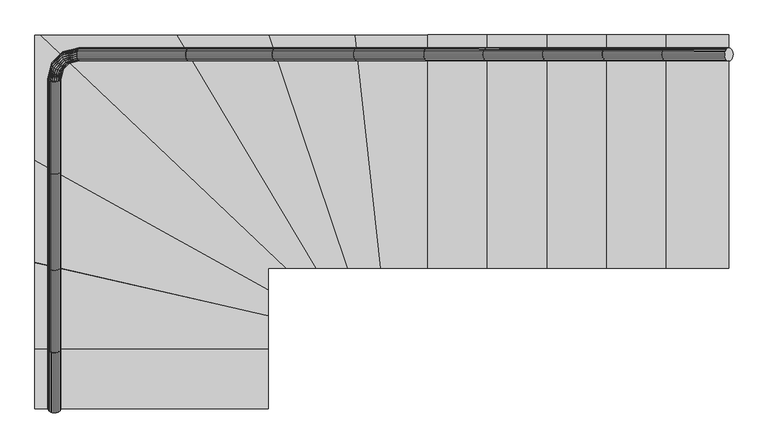
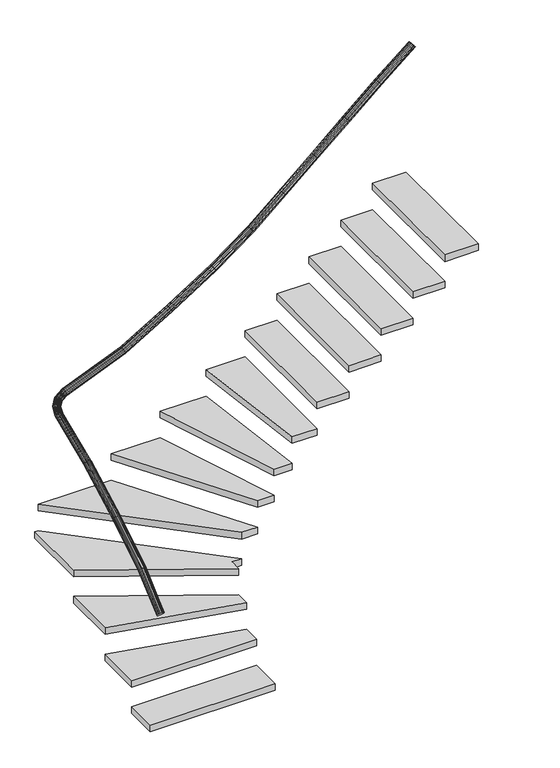
"""IFC4 building model written with IfcOpenShell, lengths in millimetres: stair geometry, 0_3d."""

from ifc_helpers import new_model, si_unit, frame, origin, origin_with_axes, place, context, project, spatial, polyline, outline, extrude, faceted_brep, source, transform, mapped, element, save


def stair_5eab08e0(model_context):
    return source(origin(), model_context, "Body", "SolidModel", [
        faceted_brep([(1247.9277886, 1358.1947934, 2262.9627611), (1243.4067036, 1356.9712063, 2269.5592366), (1238.8856187, 1358.1947934, 2276.1557121), (1234.8070891, 1361.7457815, 2282.1064787), (1231.5703496, 1367.276575, 2286.8290337), (1229.492235, 1374.2457815, 2289.8611007), (1228.7761655, 1381.9712063, 2290.9058798), (1229.492235, 1389.6966312, 2289.8611007), (1231.5703496, 1396.6658376, 2286.8290337), (1234.8070891, 1402.1966312, 2282.1064787), (1238.8856187, 1405.7476192, 2276.1557121), (1243.4067036, 1406.9712063, 2269.5592366), (1247.9277886, 1405.7476192, 2262.9627611), (1252.0063182, 1402.1966312, 2257.0119945), (1255.2430577, 1396.6658376, 2252.2894395), (1257.3211723, 1389.6966312, 2249.2573725), (1258.0372418, 1381.9712063, 2248.2125934), (1257.3211723, 1374.2457815, 2249.2573725), (1255.2430577, 1367.276575, 2252.2894395), (1252.0063182, 1361.7457815, 2257.0119945), (1509.5997401, 1358.1947934, 2475.8009775), (1514.6018366, 1356.9712063, 2469.5592366), (1519.6039331, 1358.1947934, 2463.3174957), (1524.1163895, 1361.7457815, 2457.6867399), (1527.6974952, 1367.276575, 2453.2181468), (1529.9967066, 1374.2457815, 2450.3491334), (1530.7889608, 1381.9712063, 2449.3605388), (1529.9967066, 1389.6966312, 2450.3491334), (1527.6974952, 1396.6658376, 2453.2181468), (1524.1163895, 1402.1966312, 2457.6867399), (1519.6039331, 1405.7476192, 2463.3174957), (1514.6018366, 1406.9712063, 2469.5592366), (1509.5997401, 1405.7476192, 2475.8009775), (1505.0872837, 1402.1966312, 2481.4317333), (1501.506178, 1396.6658376, 2485.9003264), (1499.2069666, 1389.6966312, 2488.7693398), (1498.4147124, 1381.9712063, 2489.7579344), (1499.2069666, 1374.2457815, 2488.7693398), (1501.506178, 1367.276575, 2485.9003264), (1505.0872837, 1361.7457815, 2481.4317333)], [[[0, 1, 2, 3, 4, 5, 6, 7, 8, 9, 10, 11, 12, 13, 14, 15, 16, 17, 18, 19]], [[20, 21, 22, 23, 24, 25, 26, 27, 28, 29, 30, 31, 32, 33, 34, 35, 36, 37, 38, 39]], [[2, 1, 21, 20]], [[3, 2, 20, 39]], [[4, 3, 39, 38]], [[5, 4, 38, 37]], [[6, 5, 37, 36]], [[7, 6, 36, 35]], [[8, 7, 35, 34]], [[9, 8, 34, 33]], [[10, 9, 33, 32]], [[11, 10, 32, 31]], [[12, 11, 31, 30]], [[13, 12, 30, 29]], [[14, 13, 29, 28]], [[15, 14, 28, 27]], [[16, 15, 27, 26]], [[17, 16, 26, 25]], [[18, 17, 25, 24]], [[19, 18, 24, 23]], [[0, 19, 23, 22]], [[1, 0, 22, 21]]]),
        extrude(outline(polyline([(1514.6018366, 1456.9712063), (1744.6018366, 1456.9712063), (1744.6018366, 556.9712063), (1514.6018366, 556.9712063), (1514.6018366, 1456.9712063)])), frame((0.0, 0.0, 1600.0), z_axis=(0.0, 0.0, 1.0), x_axis=(1.0, 0.0, 0.0)), (0.0, 0.0, 1.0), 50.0),
        extrude(outline(polyline([(0.0, 246.9712063), (0.0, 579.9383967), (900.0, 374.004016), (900.0, 246.9712063), (0.0, 246.9712063)])), frame((0.0, 0.0, 200.0), z_axis=(0.0, 0.0, 1.0), x_axis=(1.0, 0.0, 0.0)), (0.0, 0.0, 1.0), 50.0),
        extrude(outline(polyline([(2434.6018366, 1456.9712063), (2675.6316793, 1456.9712063), (2675.6316793, 556.9712063), (2434.6018366, 556.9712063), (2434.6018366, 1456.9712063)])), frame((0.0, 0.0, 2400.0), z_axis=(0.0, 0.0, 1.0), x_axis=(1.0, 0.0, 0.0)), (0.0, 0.0, 1.0), 50.0),
        extrude(outline(polyline([(548.3198618, 1456.9712063), (903.6283904, 1456.9712063), (1205.5752828, 556.9712063), (1084.8542159, 556.9712063), (548.3198618, 1456.9712063)])), frame((0.0, 0.0, 1000.0), z_axis=(0.0, 0.0, 1.0), x_axis=(1.0, 0.0, 0.0)), (0.0, 0.0, 1.0), 50.0),
        extrude(outline(polyline([(2204.6018366, 1456.9712063), (2434.6018366, 1456.9712063), (2434.6018366, 556.9712063), (2204.6018366, 556.9712063), (2204.6018366, 1456.9712063)])), frame((0.0, 0.0, 2200.0), z_axis=(0.0, 0.0, 1.0), x_axis=(1.0, 0.0, 0.0)), (0.0, 0.0, 1.0), 50.0),
        extrude(outline(polyline([(903.6283904, 1456.9712063), (1235.167677, 1456.9712063), (1334.0359962, 556.9712063), (1205.5752828, 556.9712063), (903.6283904, 1456.9712063)])), frame((0.0, 0.0, 1200.0), z_axis=(0.0, 0.0, 1.0), x_axis=(1.0, 0.0, 0.0)), (0.0, 0.0, 1.0), 50.0),
        faceted_brep([(98.7764129, 935.1107738, 1462.3430272), (100.0, 931.6520604, 1469.5592366), (98.7764129, 928.193347, 1476.775446), (95.2254249, 925.0731965, 1483.2852826), (89.6946313, 922.5970311, 1488.4515182), (82.7254249, 921.0072351, 1491.7684456), (75.0, 920.4594287, 1492.9113809), (67.2745751, 921.0072351, 1491.7684456), (60.3053687, 922.5970311, 1488.4515182), (54.7745751, 925.0731965, 1483.2852826), (51.2235871, 928.193347, 1476.775446), (50.0, 931.6520604, 1469.5592366), (51.2235871, 935.1107738, 1462.3430272), (54.7745751, 938.2309242, 1455.8331906), (60.3053687, 940.7070896, 1450.666955), (67.2745751, 942.2968856, 1447.3500276), (75.0, 942.844692, 1446.2070923), (82.7254249, 942.2968856, 1447.3500276), (89.6946313, 940.7070896, 1450.666955), (95.2254249, 938.2309242, 1455.8331906), (98.7764129, 1283.4746854, 1625.7610778), (100.0, 1286.5654708, 1618.3905793), (98.7764129, 1289.6562562, 1611.0200809), (95.2254249, 1292.4444939, 1604.3710583), (89.6946313, 1294.6572519, 1599.094364), (82.7254249, 1296.07793, 1595.7065177), (75.0, 1296.5674623, 1594.5391455), (67.2745751, 1296.07793, 1595.7065177), (60.3053687, 1294.6572519, 1599.094364), (54.7745751, 1292.4444939, 1604.3710583), (51.2235871, 1289.6562562, 1611.0200809), (50.0, 1286.5654708, 1618.3905793), (51.2235871, 1283.4746854, 1625.7610778), (54.7745751, 1280.6864477, 1632.4101004), (60.3053687, 1278.4736897, 1637.6867947), (67.2745751, 1277.0530116, 1641.074641), (75.0, 1276.5634793, 1642.2420132), (82.7254249, 1277.0530116, 1641.074641), (89.6946313, 1278.4736897, 1637.6867947), (95.2254249, 1280.6864477, 1632.4101004)], [[[0, 1, 2, 3, 4, 5, 6, 7, 8, 9, 10, 11, 12, 13, 14, 15, 16, 17, 18, 19]], [[20, 21, 22, 23, 24, 25, 26, 27, 28, 29, 30, 31, 32, 33, 34, 35, 36, 37, 38, 39]], [[2, 1, 21, 20]], [[3, 2, 20, 39]], [[4, 3, 39, 38]], [[5, 4, 38, 37]], [[6, 5, 37, 36]], [[7, 6, 36, 35]], [[8, 7, 35, 34]], [[9, 8, 34, 33]], [[10, 9, 33, 32]], [[11, 10, 32, 31]], [[12, 11, 31, 30]], [[13, 12, 30, 29]], [[14, 13, 29, 28]], [[15, 14, 28, 27]], [[16, 15, 27, 26]], [[17, 16, 26, 25]], [[18, 17, 25, 24]], [[19, 18, 24, 23]], [[0, 19, 23, 22]], [[1, 0, 22, 21]]]),
        extrude(outline(polyline([(0.0, 579.9383967), (0.0, 973.2664037), (900.0, 473.8942832), (900.0, 374.004016), (0.0, 579.9383967)])), frame((0.0, 0.0, 400.0), z_axis=(0.0, 0.0, 1.0), x_axis=(1.0, 0.0, 0.0)), (0.0, 0.0, 1.0), 50.0),
        extrude(outline(polyline([(1.2235871, -7.9923214), (0.0, 0.0), (1.2235871, 7.9923214), (4.7745752, 15.2022986), (10.3053687, 20.924169), (17.2745752, 24.5978359), (25.0, 25.8636953), (32.7254249, 24.5978359), (39.6946313, 20.924169), (45.2254249, 15.2022986), (48.7764129, 7.9923214), (50.0, 0.0), (48.7764129, -7.9923214), (45.2254249, -15.2022986), (39.6946313, -20.924169), (32.7254249, -24.5978359), (25.0, -25.8636953), (17.2745752, -24.5978359), (10.3053687, -20.924169), (4.7745752, -15.2022986), (1.2235871, -7.9923214)])), frame((1974.6018366, 1356.9712063, 2869.5592366), z_axis=(0.7546055221635011, 0.0, 0.656178714924791), x_axis=(0.0, 1.0, 0.0)), (0.0, 0.0, 1.0), 304.7950131),
        extrude(outline(polyline([(1235.167677, 1456.9712063), (1514.6018366, 1456.9712063), (1514.6018366, 556.9712063), (1334.0359962, 556.9712063), (1235.167677, 1456.9712063)])), frame((0.0, 0.0, 1400.0), z_axis=(0.0, 0.0, 1.0), x_axis=(1.0, 0.0, 0.0)), (0.0, 0.0, 1.0), 50.0),
        faceted_brep([(932.9804026, 1358.1947934, 2062.7521465), (928.7906314, 1356.9712063, 2069.5592366), (924.6008602, 1358.1947934, 2076.3663268), (920.821213, 1361.7457815, 2082.5070915), (917.821668, 1367.276575, 2087.38043), (915.8958416, 1374.2457815, 2090.5093059), (915.232247, 1381.9712063, 2091.5874431), (915.8958416, 1389.6966312, 2090.5093059), (917.821668, 1396.6658376, 2087.38043), (920.821213, 1402.1966312, 2082.5070915), (924.6008602, 1405.7476192, 2076.3663268), (928.7906314, 1406.9712063, 2069.5592366), (932.9804026, 1405.7476192, 2062.7521465), (936.7600498, 1402.1966312, 2056.6113817), (939.7595948, 1396.6658376, 2051.7380432), (941.6854212, 1389.6966312, 2048.6091673), (942.3490158, 1381.9712063, 2047.5310301), (941.6854212, 1374.2457815, 2048.6091673), (939.7595948, 1367.276575, 2051.7380432), (936.7600498, 1361.7457815, 2056.6113817), (1238.8856187, 1358.1947934, 2276.1557121), (1243.4067036, 1356.9712063, 2269.5592366), (1247.9277886, 1358.1947934, 2262.9627611), (1252.0063182, 1361.7457815, 2257.0119945), (1255.2430577, 1367.276575, 2252.2894395), (1257.3211723, 1374.2457815, 2249.2573725), (1258.0372418, 1381.9712063, 2248.2125934), (1257.3211723, 1389.6966312, 2249.2573725), (1255.2430577, 1396.6658376, 2252.2894395), (1252.0063182, 1402.1966312, 2257.0119945), (1247.9277886, 1405.7476192, 2262.9627611), (1243.4067036, 1406.9712063, 2269.5592366), (1238.8856187, 1405.7476192, 2276.1557121), (1234.8070891, 1402.1966312, 2282.1064787), (1231.5703496, 1396.6658376, 2286.8290337), (1229.492235, 1389.6966312, 2289.8611007), (1228.7761655, 1381.9712063, 2290.9058798), (1229.492235, 1374.2457815, 2289.8611007), (1231.5703496, 1367.276575, 2286.8290337), (1234.8070891, 1361.7457815, 2282.1064787)], [[[0, 1, 2, 3, 4, 5, 6, 7, 8, 9, 10, 11, 12, 13, 14, 15, 16, 17, 18, 19]], [[20, 21, 22, 23, 24, 25, 26, 27, 28, 29, 30, 31, 32, 33, 34, 35, 36, 37, 38, 39]], [[2, 1, 21, 20]], [[3, 2, 20, 39]], [[4, 3, 39, 38]], [[5, 4, 38, 37]], [[6, 5, 37, 36]], [[7, 6, 36, 35]], [[8, 7, 35, 34]], [[9, 8, 34, 33]], [[10, 9, 33, 32]], [[11, 10, 32, 31]], [[12, 11, 31, 30]], [[13, 12, 30, 29]], [[14, 13, 29, 28]], [[15, 14, 28, 27]], [[16, 15, 27, 26]], [[17, 16, 26, 25]], [[18, 17, 25, 24]], [[19, 18, 24, 23]], [[0, 19, 23, 22]], [[1, 0, 22, 21]]]),
        faceted_brep([(2439.7765349, 1358.1947934, 3263.4675843), (2434.6018366, 1356.9712063, 3269.5592366), (2429.4271383, 1358.1947934, 3275.6508889), (2424.7589754, 1361.7457815, 3281.1462478), (2421.0543005, 1367.276575, 3285.5073894), (2418.6757527, 1374.2457815, 3288.3074146), (2417.856161, 1381.9712063, 3289.2722376), (2418.6757527, 1389.6966312, 3288.3074146), (2421.0543005, 1396.6658376, 3285.5073894), (2424.7589754, 1402.1966312, 3281.1462478), (2429.4271383, 1405.7476192, 3275.6508889), (2434.6018366, 1406.9712063, 3269.5592366), (2439.7765349, 1405.7476192, 3263.4675843), (2444.4446978, 1402.1966312, 3257.9722254), (2448.1493727, 1396.6658376, 3253.6110838), (2450.5279205, 1389.6966312, 3250.8110586), (2451.3475122, 1381.9712063, 3249.8462357), (2450.5279205, 1374.2457815, 3250.8110586), (2448.1493727, 1367.276575, 3253.6110838), (2444.4446978, 1361.7457815, 3257.9722254), (2670.5280556, 1358.1947934, 3475.7098647), (2675.6316793, 1356.9712063, 3469.5592366), (2680.735303, 1358.1947934, 3463.4086085), (2685.3393485, 1361.7457815, 3457.8600467), (2688.9931396, 1367.276575, 3453.4566832), (2691.339018, 1374.2457815, 3450.6295498), (2692.1473526, 1381.9712063, 3449.655386), (2691.339018, 1389.6966312, 3450.6295498), (2688.9931396, 1396.6658376, 3453.4566832), (2685.3393485, 1402.1966312, 3457.8600467), (2680.735303, 1405.7476192, 3463.4086085), (2675.6316793, 1406.9712063, 3469.5592366), (2670.5280556, 1405.7476192, 3475.7098647), (2665.9240101, 1402.1966312, 3481.2584265), (2662.270219, 1396.6658376, 3485.66179), (2659.9243406, 1389.6966312, 3488.4889234), (2659.1160061, 1381.9712063, 3489.4630872), (2659.9243406, 1374.2457815, 3488.4889234), (2662.270219, 1367.276575, 3485.66179), (2665.9240101, 1361.7457815, 3481.2584265)], [[[0, 1, 2, 3, 4, 5, 6, 7, 8, 9, 10, 11, 12, 13, 14, 15, 16, 17, 18, 19]], [[20, 21, 22, 23, 24, 25, 26, 27, 28, 29, 30, 31, 32, 33, 34, 35, 36, 37, 38, 39]], [[2, 1, 21, 20]], [[3, 2, 20, 39]], [[4, 3, 39, 38]], [[5, 4, 38, 37]], [[6, 5, 37, 36]], [[7, 6, 36, 35]], [[8, 7, 35, 34]], [[9, 8, 34, 33]], [[10, 9, 33, 32]], [[11, 10, 32, 31]], [[12, 11, 31, 30]], [[13, 12, 30, 29]], [[14, 13, 29, 28]], [[15, 14, 28, 27]], [[16, 15, 27, 26]], [[17, 16, 26, 25]], [[18, 17, 25, 24]], [[19, 18, 24, 23]], [[0, 19, 23, 22]], [[1, 0, 22, 21]]]),
        faceted_brep([(98.7764129, 566.8246344, 1262.6622263), (100.0, 562.7771983, 1269.5592366), (98.7764129, 558.7297622, 1276.4562469), (95.2254249, 555.0785174, 1282.6781298), (89.6946313, 552.180873, 1287.615844), (82.7254249, 550.3204709, 1290.7860517), (75.0, 549.67942, 1291.8784308), (67.2745751, 550.3204709, 1290.7860517), (60.3053687, 552.180873, 1287.615844), (54.7745751, 555.0785174, 1282.6781298), (51.2235871, 558.7297622, 1276.4562469), (50.0, 562.7771983, 1269.5592366), (51.2235871, 566.8246344, 1262.6622263), (54.7745751, 570.4758792, 1256.4403434), (60.3053687, 573.3735235, 1251.5026292), (67.2745751, 575.2339257, 1248.3324215), (75.0, 575.8749766, 1247.2400424), (82.7254249, 575.2339257, 1248.3324215), (89.6946313, 573.3735235, 1251.5026292), (95.2254249, 570.4758792, 1256.4403434), (98.7764129, 928.193347, 1476.775446), (100.0, 931.6520604, 1469.5592366), (98.7764129, 935.1107738, 1462.3430272), (95.2254249, 938.2309242, 1455.8331906), (89.6946313, 940.7070896, 1450.666955), (82.7254249, 942.2968856, 1447.3500276), (75.0, 942.844692, 1446.2070923), (67.2745751, 942.2968856, 1447.3500276), (60.3053687, 940.7070896, 1450.666955), (54.7745751, 938.2309242, 1455.8331906), (51.2235871, 935.1107738, 1462.3430272), (50.0, 931.6520604, 1469.5592366), (51.2235871, 928.193347, 1476.775446), (54.7745751, 925.0731965, 1483.2852826), (60.3053687, 922.5970311, 1488.4515182), (67.2745751, 921.0072351, 1491.7684456), (75.0, 920.4594287, 1492.9113809), (82.7254249, 921.0072351, 1491.7684456), (89.6946313, 922.5970311, 1488.4515182), (95.2254249, 925.0731965, 1483.2852826)], [[[0, 1, 2, 3, 4, 5, 6, 7, 8, 9, 10, 11, 12, 13, 14, 15, 16, 17, 18, 19]], [[20, 21, 22, 23, 24, 25, 26, 27, 28, 29, 30, 31, 32, 33, 34, 35, 36, 37, 38, 39]], [[2, 1, 21, 20]], [[3, 2, 20, 39]], [[4, 3, 39, 38]], [[5, 4, 38, 37]], [[6, 5, 37, 36]], [[7, 6, 36, 35]], [[8, 7, 35, 34]], [[9, 8, 34, 33]], [[10, 9, 33, 32]], [[11, 10, 32, 31]], [[12, 11, 31, 30]], [[13, 12, 30, 29]], [[14, 13, 29, 28]], [[15, 14, 28, 27]], [[16, 15, 27, 26]], [[17, 16, 26, 25]], [[18, 17, 25, 24]], [[19, 18, 24, 23]], [[0, 19, 23, 22]], [[1, 0, 22, 21]]]),
        faceted_brep([(98.7764129, 1289.6562562, 1611.0200809), (100.0, 1286.5654708, 1618.3905793), (98.7764129, 1283.4746854, 1625.7610778), (95.2254249, 1280.6864477, 1632.4101004), (89.6946313, 1278.4736897, 1637.6867947), (82.7254249, 1277.0530116, 1641.074641), (75.0, 1276.5634793, 1642.2420132), (67.2745751, 1277.0530116, 1641.074641), (60.3053687, 1278.4736897, 1637.6867947), (54.7745751, 1280.6864477, 1632.4101004), (51.2235871, 1283.4746854, 1625.7610778), (50.0, 1286.5654708, 1618.3905793), (51.2235871, 1289.6562562, 1611.0200809), (54.7745751, 1292.4444939, 1604.3710583), (60.3053687, 1294.6572519, 1599.094364), (67.2745751, 1296.07793, 1595.7065177), (75.0, 1296.5674623, 1594.5391455), (82.7254249, 1296.07793, 1595.7065177), (89.6946313, 1294.6572519, 1599.094364), (95.2254249, 1292.4444939, 1604.3710583), (108.8478628, 1324.9929381, 1644.4685237), (105.8849612, 1322.124867, 1651.42336), (101.0649617, 1320.7116406, 1657.6974086), (94.8596795, 1320.8915954, 1662.6765216), (87.8765309, 1322.647116, 1665.873309), (80.7990751, 1325.80636, 1666.9748469), (74.3201027, 1330.0600784, 1665.873309), (69.0738208, 1334.9918878, 1662.6765216), (65.5737719, 1340.1190282, 1657.6974086), (64.1625653, 1344.9396194, 1651.42336), (64.9783397, 1348.9817884, 1644.4685237), (67.9412413, 1351.8498594, 1637.5136874), (72.7612408, 1353.2630858, 1631.2396389), (78.9665229, 1353.0831311, 1626.2605258), (85.9496716, 1351.3276104, 1623.0637384), (93.0271274, 1348.1683665, 1621.9622005), (99.5060998, 1343.914648, 1623.0637384), (104.7523817, 1338.9828387, 1626.2605258), (108.2524306, 1333.8556983, 1631.2396389), (109.6636372, 1329.0351071, 1637.5136874), (132.0400016, 1348.118589, 1672.0084164), (128.0206558, 1347.3251837, 1678.9790501), (123.2254229, 1348.7591707, 1685.2673496), (118.1236935, 1352.2801814, 1690.2577723), (113.2148606, 1357.5435547, 1693.4618209), (108.9794348, 1364.034075, 1694.5658608), (105.8320093, 1371.1164049, 1693.4618209), (104.0806759, 1378.0972767, 1690.2577723), (103.8968673, 1384.293354, 1685.2673496), (105.298576, 1389.0981215, 1678.9790501), (108.148593, 1392.0412551, 1672.0084164), (112.1679388, 1392.8346604, 1665.0377827), (116.9631718, 1391.4006734, 1658.7494833), (122.0649012, 1387.8796627, 1653.7590605), (126.9737341, 1382.6162894, 1650.5550119), (131.2091598, 1376.1257691, 1649.450972), (134.3565854, 1369.0434392, 1650.5550119), (136.1079188, 1362.0625674, 1653.7590605), (136.2917274, 1355.8664901, 1658.7494833), (134.8900186, 1351.0617226, 1665.0377827), (170.7064268, 1356.9712063, 1697.6787146), (167.6936199, 1358.1947934, 1705.08143), (164.9757274, 1361.7457815, 1711.759516), (162.8187958, 1367.276575, 1717.0592751), (161.4339604, 1374.2457815, 1720.4619299), (160.9567787, 1381.9712063, 1721.6344048), (161.4339604, 1389.6966312, 1720.4619299), (162.8187958, 1396.6658376, 1717.0592751), (164.9757274, 1402.1966312, 1711.759516), (167.6936199, 1405.7476192, 1705.08143), (170.7064268, 1406.9712063, 1697.6787146), (173.7192338, 1405.7476192, 1690.2759992), (176.4371262, 1402.1966312, 1683.5979132), (178.5940578, 1396.6658376, 1678.2981541), (179.9788932, 1389.6966312, 1674.8954993), (180.4560749, 1381.9712063, 1673.7230244), (179.9788932, 1374.2457815, 1674.8954993), (178.5940578, 1367.276575, 1678.2981541), (176.4371262, 1361.7457815, 1683.5979132), (173.7192338, 1358.1947934, 1690.2759992), (589.4593592, 1358.1947934, 1876.7344904), (593.031058, 1356.9712063, 1869.5592366), (596.6027568, 1358.1947934, 1862.3839828), (599.8248329, 1361.7457815, 1855.9110928), (602.3818869, 1367.276575, 1850.7741782), (604.0236166, 1374.2457815, 1847.476076), (604.5893182, 1381.9712063, 1846.3396275), (604.0236166, 1389.6966312, 1847.476076), (602.3818869, 1396.6658376, 1850.7741782), (599.8248329, 1402.1966312, 1855.9110928), (596.6027568, 1405.7476192, 1862.3839828), (593.031058, 1406.9712063, 1869.5592366), (589.4593592, 1405.7476192, 1876.7344904), (586.2372831, 1402.1966312, 1883.2073804), (583.6802291, 1396.6658376, 1888.344295), (582.0384994, 1389.6966312, 1891.6423972), (581.4727978, 1381.9712063, 1892.7788457), (582.0384994, 1374.2457815, 1891.6423972), (583.6802291, 1367.276575, 1888.344295), (586.2372831, 1361.7457815, 1883.2073804)], [[[0, 1, 2, 3, 4, 5, 6, 7, 8, 9, 10, 11, 12, 13, 14, 15, 16, 17, 18, 19]], [[2, 1, 20]], [[21, 2, 20]], [[3, 2, 21]], [[22, 3, 21]], [[4, 3, 22]], [[23, 4, 22]], [[5, 4, 23]], [[24, 5, 23]], [[6, 5, 24]], [[25, 6, 24]], [[7, 6, 25]], [[26, 7, 25]], [[8, 7, 26]], [[27, 8, 26]], [[9, 8, 27]], [[28, 9, 27]], [[10, 9, 28]], [[29, 10, 28]], [[11, 10, 29]], [[30, 11, 29]], [[12, 11, 30]], [[31, 12, 30]], [[13, 12, 31]], [[32, 13, 31]], [[14, 13, 32]], [[33, 14, 32]], [[15, 14, 33]], [[34, 15, 33]], [[16, 15, 34]], [[35, 16, 34]], [[17, 16, 35]], [[36, 17, 35]], [[18, 17, 36]], [[37, 18, 36]], [[19, 18, 37]], [[38, 19, 37]], [[0, 19, 38]], [[39, 0, 38]], [[1, 0, 39]], [[20, 1, 39]], [[21, 20, 40]], [[41, 21, 40]], [[22, 21, 41]], [[42, 22, 41]], [[23, 22, 42]], [[43, 23, 42]], [[24, 23, 43]], [[44, 24, 43]], [[25, 24, 44]], [[45, 25, 44]], [[26, 25, 45]], [[46, 26, 45]], [[27, 26, 46]], [[47, 27, 46]], [[28, 27, 47]], [[48, 28, 47]], [[29, 28, 48]], [[49, 29, 48]], [[30, 29, 49]], [[50, 30, 49]], [[31, 30, 50]], [[51, 31, 50]], [[32, 31, 51]], [[52, 32, 51]], [[33, 32, 52]], [[53, 33, 52]], [[34, 33, 53]], [[54, 34, 53]], [[35, 34, 54]], [[55, 35, 54]], [[36, 35, 55]], [[56, 36, 55]], [[37, 36, 56]], [[57, 37, 56]], [[38, 37, 57]], [[58, 38, 57]], [[39, 38, 58]], [[59, 39, 58]], [[20, 39, 59]], [[40, 20, 59]], [[41, 40, 60]], [[61, 41, 60]], [[42, 41, 61]], [[62, 42, 61]], [[43, 42, 62]], [[63, 43, 62]], [[44, 43, 63]], [[64, 44, 63]], [[45, 44, 64]], [[65, 45, 64]], [[46, 45, 65]], [[66, 46, 65]], [[47, 46, 66]], [[67, 47, 66]], [[48, 47, 67]], [[68, 48, 67]], [[49, 48, 68]], [[69, 49, 68]], [[50, 49, 69]], [[70, 50, 69]], [[51, 50, 70]], [[71, 51, 70]], [[52, 51, 71]], [[72, 52, 71]], [[53, 52, 72]], [[73, 53, 72]], [[54, 53, 73]], [[74, 54, 73]], [[55, 54, 74]], [[75, 55, 74]], [[56, 55, 75]], [[76, 56, 75]], [[57, 56, 76]], [[77, 57, 76]], [[58, 57, 77]], [[78, 58, 77]], [[59, 58, 78]], [[79, 59, 78]], [[40, 59, 79]], [[60, 40, 79]], [[80, 81, 82, 83, 84, 85, 86, 87, 88, 89, 90, 91, 92, 93, 94, 95, 96, 97, 98, 99]], [[61, 60, 81, 80]], [[62, 61, 80, 99]], [[63, 62, 99, 98]], [[64, 63, 98, 97]], [[65, 64, 97, 96]], [[66, 65, 96, 95]], [[67, 66, 95, 94]], [[68, 67, 94, 93]], [[69, 68, 93, 92]], [[70, 69, 92, 91]], [[71, 70, 91, 90]], [[72, 71, 90, 89]], [[73, 72, 89, 88]], [[74, 73, 88, 87]], [[75, 74, 87, 86]], [[76, 75, 86, 85]], [[77, 76, 85, 84]], [[78, 77, 84, 83]], [[79, 78, 83, 82]], [[60, 79, 82, 81]]]),
        faceted_brep([(596.6027568, 1358.1947934, 1862.3839828), (593.031058, 1356.9712063, 1869.5592366), (589.4593592, 1358.1947934, 1876.7344904), (586.2372831, 1361.7457815, 1883.2073804), (583.6802291, 1367.276575, 1888.344295), (582.0384994, 1374.2457815, 1891.6423972), (581.4727978, 1381.9712063, 1892.7788457), (582.0384994, 1389.6966312, 1891.6423972), (583.6802291, 1396.6658376, 1888.344295), (586.2372831, 1402.1966312, 1883.2073804), (589.4593592, 1405.7476192, 1876.7344904), (593.031058, 1406.9712063, 1869.5592366), (596.6027568, 1405.7476192, 1862.3839828), (599.8248329, 1402.1966312, 1855.9110928), (602.3818869, 1396.6658376, 1850.7741782), (604.0236166, 1389.6966312, 1847.476076), (604.5893182, 1381.9712063, 1846.3396275), (604.0236166, 1374.2457815, 1847.476076), (602.3818869, 1367.276575, 1850.7741782), (599.8248329, 1361.7457815, 1855.9110928), (924.6008602, 1358.1947934, 2076.3663268), (928.7906314, 1356.9712063, 2069.5592366), (932.9804026, 1358.1947934, 2062.7521465), (936.7600498, 1361.7457815, 2056.6113817), (939.7595948, 1367.276575, 2051.7380432), (941.6854212, 1374.2457815, 2048.6091673), (942.3490158, 1381.9712063, 2047.5310301), (941.6854212, 1389.6966312, 2048.6091673), (939.7595948, 1396.6658376, 2051.7380432), (936.7600498, 1402.1966312, 2056.6113817), (932.9804026, 1405.7476192, 2062.7521465), (928.7906314, 1406.9712063, 2069.5592366), (924.6008602, 1405.7476192, 2076.3663268), (920.821213, 1402.1966312, 2082.5070915), (917.821668, 1396.6658376, 2087.38043), (915.8958416, 1389.6966312, 2090.5093059), (915.232247, 1381.9712063, 2091.5874431), (915.8958416, 1374.2457815, 2090.5093059), (917.821668, 1367.276575, 2087.38043), (920.821213, 1361.7457815, 2082.5070915)], [[[0, 1, 2, 3, 4, 5, 6, 7, 8, 9, 10, 11, 12, 13, 14, 15, 16, 17, 18, 19]], [[20, 21, 22, 23, 24, 25, 26, 27, 28, 29, 30, 31, 32, 33, 34, 35, 36, 37, 38, 39]], [[2, 1, 21, 20]], [[3, 2, 20, 39]], [[4, 3, 39, 38]], [[5, 4, 38, 37]], [[6, 5, 37, 36]], [[7, 6, 36, 35]], [[8, 7, 35, 34]], [[9, 8, 34, 33]], [[10, 9, 33, 32]], [[11, 10, 32, 31]], [[12, 11, 31, 30]], [[13, 12, 30, 29]], [[14, 13, 29, 28]], [[15, 14, 28, 27]], [[16, 15, 27, 26]], [[17, 16, 26, 25]], [[18, 17, 25, 24]], [[19, 18, 24, 23]], [[0, 19, 23, 22]], [[1, 0, 22, 21]]]),
        faceted_brep([(98.7764129, 22.2155975, 863.5281868), (100.0, 16.9712063, 869.5592366), (98.7764129, 11.7268152, 875.5902865), (95.2254249, 6.9957815, 881.0309751), (89.6946313, 3.241212, 885.3487301), (82.7254249, 0.83063, 888.1208994), (75.0, 0.0, 889.0761239), (67.2745751, 0.83063, 888.1208994), (60.3053687, 3.241212, 885.3487301), (54.7745751, 6.9957815, 881.0309751), (51.2235871, 11.7268152, 875.5902865), (50.0, 16.9712063, 869.5592366), (51.2235871, 22.2155975, 863.5281868), (54.7745751, 26.9466311, 858.0874981), (60.3053687, 30.7012007, 853.7697431), (67.2745751, 33.1117827, 850.9975738), (75.0, 33.9424127, 850.0423493), (82.7254249, 33.1117827, 850.9975738), (89.6946313, 30.7012007, 853.7697431), (95.2254249, 26.9466311, 858.0874981), (98.7764129, 242.1836266, 1075.9875138), (100.0, 246.9712063, 1069.5592366), (98.7764129, 251.7587861, 1063.1309594), (95.2254249, 256.0777241, 1057.3319268), (89.6946313, 259.5052528, 1052.7297884), (82.7254249, 261.7058616, 1049.7750337), (75.0, 262.4641398, 1048.7568947), (67.2745751, 261.7058616, 1049.7750337), (60.3053687, 259.5052528, 1052.7297884), (54.7745751, 256.0777241, 1057.3319268), (51.2235871, 251.7587861, 1063.1309594), (50.0, 246.9712063, 1069.5592366), (51.2235871, 242.1836266, 1075.9875138), (54.7745751, 237.8646885, 1081.7865464), (60.3053687, 234.4371599, 1086.3886848), (67.2745751, 232.236551, 1089.3434395), (75.0, 231.4782729, 1090.3615786), (82.7254249, 232.236551, 1089.3434395), (89.6946313, 234.4371599, 1086.3886848), (95.2254249, 237.8646885, 1081.7865464)], [[[0, 1, 2, 3, 4, 5, 6, 7, 8, 9, 10, 11, 12, 13, 14, 15, 16, 17, 18, 19]], [[20, 21, 22, 23, 24, 25, 26, 27, 28, 29, 30, 31, 32, 33, 34, 35, 36, 37, 38, 39]], [[2, 1, 21, 20]], [[3, 2, 20, 39]], [[4, 3, 39, 38]], [[5, 4, 38, 37]], [[6, 5, 37, 36]], [[7, 6, 36, 35]], [[8, 7, 35, 34]], [[9, 8, 34, 33]], [[10, 9, 33, 32]], [[11, 10, 32, 31]], [[12, 11, 31, 30]], [[13, 12, 30, 29]], [[14, 13, 29, 28]], [[15, 14, 28, 27]], [[16, 15, 27, 26]], [[17, 16, 26, 25]], [[18, 17, 25, 24]], [[19, 18, 24, 23]], [[0, 19, 23, 22]], [[1, 0, 22, 21]]]),
        extrude(outline(polyline([(0.0, 16.9712063), (0.0, 246.9712063), (900.0, 246.9712063), (900.0, 16.9712063), (0.0, 16.9712063)])), origin_with_axes(), (0.0, 0.0, 1.0), 50.0),
        extrude(outline(polyline([(1.2235871, -7.9923214), (0.0, 0.0), (1.2235871, 7.9923214), (4.7745752, 15.2022986), (10.3053687, 20.924169), (17.2745752, 24.5978359), (25.0, 25.8636953), (32.7254249, 24.5978359), (39.6946313, 20.924169), (45.2254249, 15.2022986), (48.7764129, 7.9923214), (50.0, 0.0), (48.7764129, -7.9923214), (45.2254249, -15.2022986), (39.6946313, -20.924169), (32.7254249, -24.5978359), (25.0, -25.8636953), (17.2745752, -24.5978359), (10.3053687, -20.924169), (4.7745752, -15.2022986), (1.2235871, -7.9923214)])), frame((1744.6018366, 1356.9712063, 2669.5592366), z_axis=(0.7546055221634738, 0.0, 0.6561787149248223), x_axis=(0.0, 1.0, 0.0)), (0.0, 0.0, 1.0), 304.7950131),
        faceted_brep([(1519.6039331, 1358.1947934, 2463.3174957), (1514.6018366, 1356.9712063, 2469.5592366), (1509.5997401, 1358.1947934, 2475.8009775), (1505.0872837, 1361.7457815, 2481.4317333), (1501.506178, 1367.276575, 2485.9003264), (1499.2069666, 1374.2457815, 2488.7693398), (1498.4147124, 1381.9712063, 2489.7579344), (1499.2069666, 1389.6966312, 2488.7693398), (1501.506178, 1396.6658376, 2485.9003264), (1505.0872837, 1402.1966312, 2481.4317333), (1509.5997401, 1405.7476192, 2475.8009775), (1514.6018366, 1406.9712063, 2469.5592366), (1519.6039331, 1405.7476192, 2463.3174957), (1524.1163895, 1402.1966312, 2457.6867399), (1527.6974952, 1396.6658376, 2453.2181468), (1529.9967066, 1389.6966312, 2450.3491334), (1530.7889608, 1381.9712063, 2449.3605388), (1529.9967066, 1374.2457815, 2450.3491334), (1527.6974952, 1367.276575, 2453.2181468), (1524.1163895, 1361.7457815, 2457.6867399), (1739.3574454, 1358.1947934, 2675.5902865), (1744.6018366, 1356.9712063, 2669.5592366), (1749.8462278, 1358.1947934, 2663.5281868), (1754.5772614, 1361.7457815, 2658.0874981), (1758.3318309, 1367.276575, 2653.7697431), (1760.742413, 1374.2457815, 2650.9975738), (1761.5730429, 1381.9712063, 2650.0423493), (1760.742413, 1389.6966312, 2650.9975738), (1758.3318309, 1396.6658376, 2653.7697431), (1754.5772614, 1402.1966312, 2658.0874981), (1749.8462278, 1405.7476192, 2663.5281868), (1744.6018366, 1406.9712063, 2669.5592366), (1739.3574454, 1405.7476192, 2675.5902865), (1734.6264118, 1402.1966312, 2681.0309751), (1730.8718423, 1396.6658376, 2685.3487301), (1728.4612602, 1389.6966312, 2688.1208994), (1727.6306303, 1381.9712063, 2689.0761239), (1728.4612602, 1374.2457815, 2688.1208994), (1730.8718423, 1367.276575, 2685.3487301), (1734.6264118, 1361.7457815, 2681.0309751)], [[[0, 1, 2, 3, 4, 5, 6, 7, 8, 9, 10, 11, 12, 13, 14, 15, 16, 17, 18, 19]], [[20, 21, 22, 23, 24, 25, 26, 27, 28, 29, 30, 31, 32, 33, 34, 35, 36, 37, 38, 39]], [[2, 1, 21, 20]], [[3, 2, 20, 39]], [[4, 3, 39, 38]], [[5, 4, 38, 37]], [[6, 5, 37, 36]], [[7, 6, 36, 35]], [[8, 7, 35, 34]], [[9, 8, 34, 33]], [[10, 9, 33, 32]], [[11, 10, 32, 31]], [[12, 11, 31, 30]], [[13, 12, 30, 29]], [[14, 13, 29, 28]], [[15, 14, 28, 27]], [[16, 15, 27, 26]], [[17, 16, 26, 25]], [[18, 17, 25, 24]], [[19, 18, 24, 23]], [[0, 19, 23, 22]], [[1, 0, 22, 21]]]),
        faceted_brep([(98.7764129, 251.7587861, 1063.1309594), (100.0, 246.9712063, 1069.5592366), (98.7764129, 242.1836266, 1075.9875138), (95.2254249, 237.8646885, 1081.7865464), (89.6946313, 234.4371599, 1086.3886848), (82.7254249, 232.236551, 1089.3434395), (75.0, 231.4782729, 1090.3615786), (67.2745751, 232.236551, 1089.3434395), (60.3053687, 234.4371599, 1086.3886848), (54.7745751, 237.8646885, 1081.7865464), (51.2235871, 242.1836266, 1075.9875138), (50.0, 246.9712063, 1069.5592366), (51.2235871, 251.7587861, 1063.1309594), (54.7745751, 256.0777241, 1057.3319268), (60.3053687, 259.5052528, 1052.7297884), (67.2745751, 261.7058616, 1049.7750337), (75.0, 262.4641398, 1048.7568947), (82.7254249, 261.7058616, 1049.7750337), (89.6946313, 259.5052528, 1052.7297884), (95.2254249, 256.0777241, 1057.3319268), (98.7764129, 558.7297622, 1276.4562469), (100.0, 562.7771983, 1269.5592366), (98.7764129, 566.8246344, 1262.6622263), (95.2254249, 570.4758792, 1256.4403434), (89.6946313, 573.3735235, 1251.5026292), (82.7254249, 575.2339257, 1248.3324215), (75.0, 575.8749766, 1247.2400424), (67.2745751, 575.2339257, 1248.3324215), (60.3053687, 573.3735235, 1251.5026292), (54.7745751, 570.4758792, 1256.4403434), (51.2235871, 566.8246344, 1262.6622263), (50.0, 562.7771983, 1269.5592366), (51.2235871, 558.7297622, 1276.4562469), (54.7745751, 555.0785174, 1282.6781298), (60.3053687, 552.180873, 1287.615844), (67.2745751, 550.3204709, 1290.7860517), (75.0, 549.67942, 1291.8784308), (82.7254249, 550.3204709, 1290.7860517), (89.6946313, 552.180873, 1287.615844), (95.2254249, 555.0785174, 1282.6781298)], [[[0, 1, 2, 3, 4, 5, 6, 7, 8, 9, 10, 11, 12, 13, 14, 15, 16, 17, 18, 19]], [[20, 21, 22, 23, 24, 25, 26, 27, 28, 29, 30, 31, 32, 33, 34, 35, 36, 37, 38, 39]], [[2, 1, 21, 20]], [[3, 2, 20, 39]], [[4, 3, 39, 38]], [[5, 4, 38, 37]], [[6, 5, 37, 36]], [[7, 6, 36, 35]], [[8, 7, 35, 34]], [[9, 8, 34, 33]], [[10, 9, 33, 32]], [[11, 10, 32, 31]], [[12, 11, 31, 30]], [[13, 12, 30, 29]], [[14, 13, 29, 28]], [[15, 14, 28, 27]], [[16, 15, 27, 26]], [[17, 16, 26, 25]], [[18, 17, 25, 24]], [[19, 18, 24, 23]], [[0, 19, 23, 22]], [[1, 0, 22, 21]]]),
        extrude(outline(polyline([(1974.6018366, 1456.9712063), (2204.6018366, 1456.9712063), (2204.6018366, 556.9712063), (1974.6018366, 556.9712063), (1974.6018366, 1456.9712063)])), frame((0.0, 0.0, 2000.0), z_axis=(0.0, 0.0, 1.0), x_axis=(1.0, 0.0, 0.0)), (0.0, 0.0, 1.0), 50.0),
        extrude(outline(polyline([(1744.6018366, 1456.9712063), (1974.6018366, 1456.9712063), (1974.6018366, 556.9712063), (1744.6018366, 556.9712063), (1744.6018366, 1456.9712063)])), frame((0.0, 0.0, 1800.0), z_axis=(0.0, 0.0, 1.0), x_axis=(1.0, 0.0, 0.0)), (0.0, 0.0, 1.0), 50.0),
        faceted_brep([(2209.8462278, 1358.1947934, 3063.5281868), (2204.6018366, 1356.9712063, 3069.5592366), (2199.3574454, 1358.1947934, 3075.5902865), (2194.6264118, 1361.7457815, 3081.0309751), (2190.8718423, 1367.276575, 3085.3487301), (2188.4612602, 1374.2457815, 3088.1208994), (2187.6306303, 1381.9712063, 3089.0761239), (2188.4612602, 1389.6966312, 3088.1208994), (2190.8718423, 1396.6658376, 3085.3487301), (2194.6264118, 1402.1966312, 3081.0309751), (2199.3574454, 1405.7476192, 3075.5902865), (2204.6018366, 1406.9712063, 3069.5592366), (2209.8462278, 1405.7476192, 3063.5281868), (2214.5772614, 1402.1966312, 3058.0874981), (2218.3318309, 1396.6658376, 3053.7697431), (2220.742413, 1389.6966312, 3050.9975738), (2221.5730429, 1381.9712063, 3050.0423493), (2220.742413, 1374.2457815, 3050.9975738), (2218.3318309, 1367.276575, 3053.7697431), (2214.5772614, 1361.7457815, 3058.0874981), (2429.4271383, 1358.1947934, 3275.6508889), (2434.6018366, 1356.9712063, 3269.5592366), (2439.7765349, 1358.1947934, 3263.4675843), (2444.4446978, 1361.7457815, 3257.9722254), (2448.1493727, 1367.276575, 3253.6110838), (2450.5279205, 1374.2457815, 3250.8110586), (2451.3475122, 1381.9712063, 3249.8462357), (2450.5279205, 1389.6966312, 3250.8110586), (2448.1493727, 1396.6658376, 3253.6110838), (2444.4446978, 1402.1966312, 3257.9722254), (2439.7765349, 1405.7476192, 3263.4675843), (2434.6018366, 1406.9712063, 3269.5592366), (2429.4271383, 1405.7476192, 3275.6508889), (2424.7589754, 1402.1966312, 3281.1462478), (2421.0543005, 1396.6658376, 3285.5073894), (2418.6757527, 1389.6966312, 3288.3074146), (2417.856161, 1381.9712063, 3289.2722376), (2418.6757527, 1374.2457815, 3288.3074146), (2421.0543005, 1367.276575, 3285.5073894), (2424.7589754, 1361.7457815, 3281.1462478)], [[[0, 1, 2, 3, 4, 5, 6, 7, 8, 9, 10, 11, 12, 13, 14, 15, 16, 17, 18, 19]], [[20, 21, 22, 23, 24, 25, 26, 27, 28, 29, 30, 31, 32, 33, 34, 35, 36, 37, 38, 39]], [[2, 1, 21, 20]], [[3, 2, 20, 39]], [[4, 3, 39, 38]], [[5, 4, 38, 37]], [[6, 5, 37, 36]], [[7, 6, 36, 35]], [[8, 7, 35, 34]], [[9, 8, 34, 33]], [[10, 9, 33, 32]], [[11, 10, 32, 31]], [[12, 11, 31, 30]], [[13, 12, 30, 29]], [[14, 13, 29, 28]], [[15, 14, 28, 27]], [[16, 15, 27, 26]], [[17, 16, 26, 25]], [[18, 17, 25, 24]], [[19, 18, 24, 23]], [[0, 19, 23, 22]], [[1, 0, 22, 21]]]),
        extrude(outline(polyline([(22.6704161, 1456.9712063), (548.3198618, 1456.9712063), (1084.8542159, 556.9712063), (970.0, 556.9712063), (22.6704161, 1456.9712063)])), frame((0.0, 0.0, 800.0), z_axis=(0.0, 0.0, 1.0), x_axis=(1.0, 0.0, 0.0)), (0.0, 0.0, 1.0), 50.0),
        extrude(outline(polyline([(0.0, 973.2664037), (0.0, 1456.9712063), (22.6704161, 1456.9712063), (970.0, 556.9712063), (900.0, 556.9712063), (900.0, 473.8942832), (0.0, 973.2664037)])), frame((0.0, 0.0, 600.0), z_axis=(0.0, 0.0, 1.0), x_axis=(1.0, 0.0, 0.0)), (0.0, 0.0, 1.0), 50.0),
    ])


if __name__ == "__main__":
    model = new_model("IFC4")
    model_context = context("Model", 3, world=origin())
    ifc_project = project(units=[si_unit("LENGTHUNIT", "METRE", prefix="MILLI")], contexts=[model_context])
    site = spatial("IfcSite", under=ifc_project)
    building = spatial("IfcBuilding", under=site)
    placement = place(None, origin())
    stair_shape = stair_5eab08e0(model_context)
    element("IfcStair", 1, ObjectType="0_3d", at=placement, inside=building, context=model_context, shape_type="MappedRepresentation", body=[
        mapped(stair_shape, transform((0.0, 0.0, 0.0), x_axis=(1.0, 0.0, 0.0), y_axis=(0.0, 1.0, 0.0), z_axis=(0.0, 0.0, 1.0))),
    ])
    save(model, "model.ifc")

# Revit data of these elements
# Element 1 (IfcStair, "0_3d")
#   Materials on its faces: "*1", "weiss"
# Materials
#   "*1": class "Unassigned", colour RGB 175 175 175, transparency 0
#   "weiss": class "Unassigned", colour RGB 255 255 255, transparency 0
